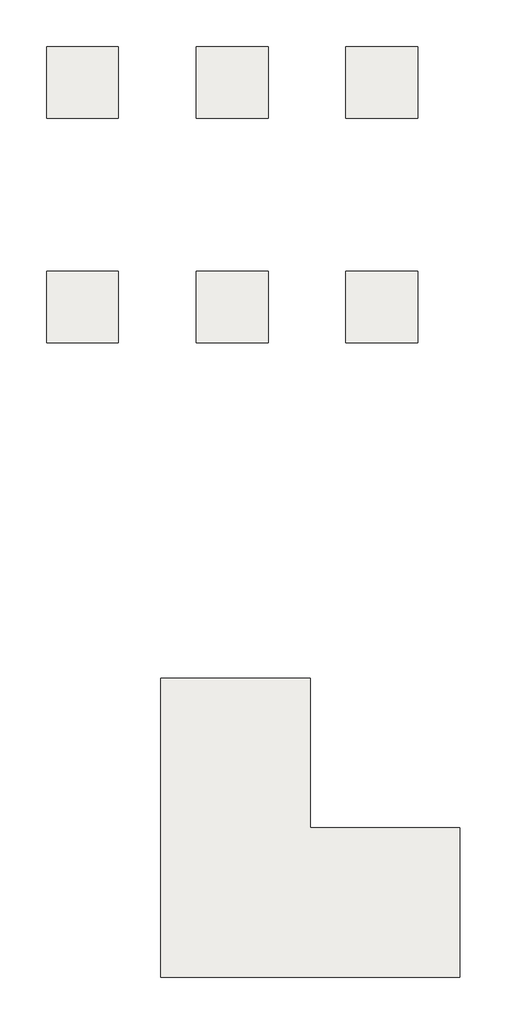
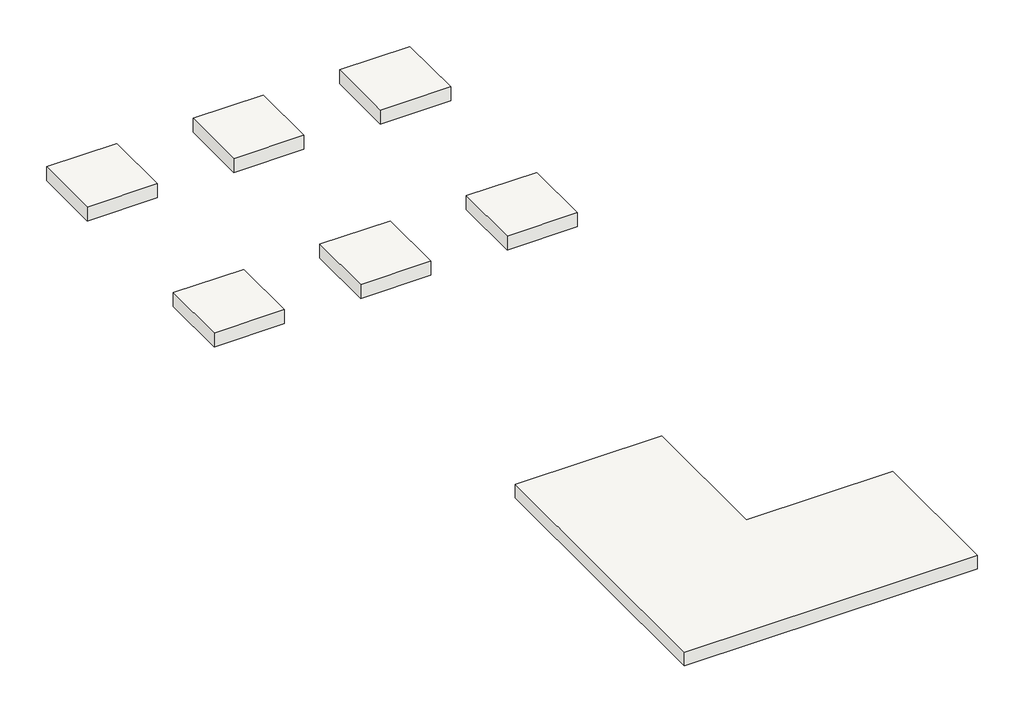
# Not in any storey: 7 slabs.
"""IFC4 building model written with IfcOpenShell, lengths in millimetres."""

import ifcopenshell
import ifcopenshell.guid

model = None  # the IFC model being written
_history = None  # IfcOwnerHistory: only IFC2X3 demands one
_inside = {}  # id of a spatial element -> (the spatial element, [elements in it])
_under = {}  # id of a project, library or spatial element -> (it, [spatial elements below it])
_declared = {}  # id of a project -> (the project, [libraries it declares])
_typed = {}  # id of a type object -> (the type object, [elements of that type])
_made_of = {}  # id of a material, layer set ... -> (it, [elements and type objects made of it])


def new_model(schema):
    """Start an empty IFC model of exactly this schema.

    Asked for "IFC4X3", IfcOpenShell would pick the latest addendum, in which some entities
    have other attributes; the version numbers below select the first issue.
    IFC2X3 requires an IfcOwnerHistory on every rooted entity: one is made here for all.
    """
    global model, _history
    if schema == "IFC4X3":
        model = ifcopenshell.file(schema_version=(4, 3, 0, 0))
    else:
        model = ifcopenshell.file(schema=schema)
    _inside.clear()
    _under.clear()
    _declared.clear()
    _typed.clear()
    _made_of.clear()
    _history = None
    if model.schema == "IFC2X3":
        org = make("IfcOrganization", Name="unknown")
        user = make(
            "IfcPersonAndOrganization",
            ThePerson=make("IfcPerson", FamilyName="unknown"),
            TheOrganization=org,
        )
        app = make(
            "IfcApplication",
            ApplicationDeveloper=org,
            Version="unknown",
            ApplicationFullName="unknown",
            ApplicationIdentifier="unknown",
        )
        _history = make(
            "IfcOwnerHistory",
            OwningUser=user,
            OwningApplication=app,
            ChangeAction="ADDED",
            CreationDate=0,
        )
    return model


def make(cls, **values):
    """One entity of the class cls with the attributes given. An attribute that is None is left unset."""
    return model.create_entity(
        cls, **{name: value for name, value in values.items() if value is not None}
    )


def rooted(cls, **values):
    """An entity with a GlobalId (a new one), such as an element, a storey or a relation."""
    return make(cls, GlobalId=ifcopenshell.guid.new(), OwnerHistory=_history, **values)


def si_unit(unit_type, name, prefix=None):
    """IfcSIUnit, for example si_unit("LENGTHUNIT", "METRE", prefix="MILLI")."""
    return make("IfcSIUnit", UnitType=unit_type, Prefix=prefix, Name=name)


def assignment(units):
    """IfcUnitAssignment: the units of a project."""
    return None if units is None else make("IfcUnitAssignment", Units=units)


def point(xyz):
    """IfcCartesianPoint."""
    return None if xyz is None else make("IfcCartesianPoint", Coordinates=xyz)


def direction(xyz):
    """IfcDirection."""
    return None if xyz is None else make("IfcDirection", DirectionRatios=xyz)


def frame(location, z_axis=None, x_axis=None):
    """IfcAxis2Placement3D, a coordinate frame: its origin and axes. An axis left out is left unset."""
    return make(
        "IfcAxis2Placement3D",
        Location=point(location),
        Axis=direction(z_axis),
        RefDirection=direction(x_axis),
    )


def origin():
    """The frame at (0, 0, 0) with its axes left unset."""
    return frame((0.0, 0.0, 0.0))


def place(relative_to, where):
    """IfcLocalPlacement: puts the frame where relative to a parent placement (None: the world)."""
    return make(
        "IfcLocalPlacement", PlacementRelTo=relative_to, RelativePlacement=where
    )


def context(
    kind, dimensions, precision=None, world=None, true_north=None, identifier=None
):
    """IfcGeometricRepresentationContext, for example the 3D "Model" context."""
    return make(
        "IfcGeometricRepresentationContext",
        ContextIdentifier=identifier,
        ContextType=kind,
        CoordinateSpaceDimension=dimensions,
        Precision=precision,
        WorldCoordinateSystem=world,
        TrueNorth=true_north,
    )


def project(units=None, contexts=None):
    """IfcProject with its units and contexts."""
    return rooted(
        "IfcProject",
        Name="project",
        RepresentationContexts=contexts,
        UnitsInContext=assignment(units),
    )


def spatial(cls, under=None, at=None, **own):
    """A site, building, storey or space (cls), placed at a placement, below another one or the project."""
    s = rooted(cls, ObjectPlacement=at, **own)
    if under is not None:
        _under.setdefault(under.id(), (under, []))[1].append(s)
    return s


def polyline(points):
    """IfcPolyline through the points."""
    return make("IfcPolyline", Points=[point(p) for p in points])


def outline(outer, holes=None, kind="AREA"):
    """IfcArbitraryClosedProfileDef: a profile drawn as a closed curve; with holes, ...WithVoids."""
    if holes is None:
        return make("IfcArbitraryClosedProfileDef", ProfileType=kind, OuterCurve=outer)
    return make(
        "IfcArbitraryProfileDefWithVoids",
        ProfileType=kind,
        OuterCurve=outer,
        InnerCurves=holes,
    )


def extrude(swept, where, along, depth):
    """IfcExtrudedAreaSolid: the profile swept, set in the frame where, extruded along a direction by depth."""
    return make(
        "IfcExtrudedAreaSolid",
        SweptArea=swept,
        Position=where,
        ExtrudedDirection=direction(along),
        Depth=depth,
    )


def shape(context_of_items, identifier, shape_type, items):
    """IfcShapeRepresentation: the items that make up one representation, for example the "Body"."""
    return make(
        "IfcShapeRepresentation",
        ContextOfItems=context_of_items,
        RepresentationIdentifier=identifier,
        RepresentationType=shape_type,
        Items=items,
    )


def source(mapping_origin, context_of_items, identifier, shape_type, items):
    """IfcRepresentationMap: a shape defined once, which mapped items show again and again."""
    return make(
        "IfcRepresentationMap",
        MappingOrigin=mapping_origin,
        MappedRepresentation=shape(context_of_items, identifier, shape_type, items),
    )


def transform(
    local_origin,
    x_axis=None,
    y_axis=None,
    z_axis=None,
    scale=None,
    scale2=None,
    scale3=None,
    uniform=True,
):
    """IfcCartesianTransformationOperator3D, or its non-uniform kind. x_axis, y_axis, z_axis: its Axis1, 2, 3."""
    if uniform:
        return make(
            "IfcCartesianTransformationOperator3D",
            Axis1=direction(x_axis),
            Axis2=direction(y_axis),
            LocalOrigin=point(local_origin),
            Scale=scale,
            Axis3=direction(z_axis),
        )
    return make(
        "IfcCartesianTransformationOperator3DnonUniform",
        Axis1=direction(x_axis),
        Axis2=direction(y_axis),
        LocalOrigin=point(local_origin),
        Scale=scale,
        Axis3=direction(z_axis),
        Scale2=scale2,
        Scale3=scale3,
    )


def mapped(mapping_source, mapping_target):
    """IfcMappedItem: shows the shape of a source again, moved by a transform."""
    return make(
        "IfcMappedItem", MappingSource=mapping_source, MappingTarget=mapping_target
    )


def made_of(thing, what):
    """Note that an element or type object is made of a material, layer set ...; save() writes the relation."""
    if what is not None:
        _made_of.setdefault(what.id(), (what, []))[1].append(thing)
    return thing


def element(
    cls,
    number,
    at=None,
    inside=None,
    cuts=None,
    type_object=None,
    material=None,
    context=None,
    identifier="Body",
    shape_type=None,
    held_by="IfcProductDefinitionShape",
    body=None,
    shapes=None,
    **own,
):
    """One element of the class cls, such as IfcWall. Its Tag is "e" and its number.

    at: its placement. inside: the storey or other place that contains it. cuts: it is an
    opening in that element (IfcRelVoidsElement). A single representation is given by context,
    identifier, shape_type and body (its items); several are given by shapes. held_by: the class
    of the entity that holds the representations. save() writes the other relations.
    """
    e = rooted(cls, Tag="e%d" % number, ObjectPlacement=at, **own)
    if body is not None:
        shapes = [shape(context, identifier, shape_type, body)]
    if shapes is not None:
        e.Representation = make(held_by, Representations=shapes)
    if inside is not None:
        _inside.setdefault(inside.id(), (inside, []))[1].append(e)
    if cuts is not None:
        rooted(
            "IfcRelVoidsElement", RelatingBuildingElement=cuts, RelatedOpeningElement=e
        )
    if type_object is not None:
        _typed.setdefault(type_object.id(), (type_object, []))[1].append(e)
    return made_of(e, material)


def aggregate(whole, parts):
    """IfcRelAggregates: a whole, such as a stair, and the parts it consists of."""
    return rooted("IfcRelAggregates", RelatingObject=whole, RelatedObjects=parts)


def save(model, path):
    """Write the relations noted so far, then the file.

    IfcRelAggregates (storeys below a building ...), IfcRelContainedInSpatialStructure (elements
    in a storey), IfcRelDefinesByType, IfcRelAssociatesMaterial and IfcRelDeclares: one each for
    every whole, place, type object, material and project.
    """
    for whole, parts in _under.values():
        aggregate(whole, parts)
    for where, things in _inside.values():
        rooted(
            "IfcRelContainedInSpatialStructure",
            RelatedElements=things,
            RelatingStructure=where,
        )
    for kind, things in _typed.values():
        rooted("IfcRelDefinesByType", RelatedObjects=things, RelatingType=kind)
    for what, things in _made_of.values():
        rooted("IfcRelAssociatesMaterial", RelatedObjects=things, RelatingMaterial=what)
    for by, libraries in _declared.values():
        rooted("IfcRelDeclares", RelatingContext=by, RelatedDefinitions=libraries)
    model.write(path)


def ft211_footing_rectangular_void_test_ft211_10000x10000x500_68336e3b(model_context):
    return source(origin(), model_context, "Body", "SweptSolid", [
        extrude(outline(polyline([(5000.0, -5000.0), (-5000.0, -5000.0), (-5000.0, 5000.0), (0.0, 5000.0), (0.0, 0.0), (5000.0, 0.0), (5000.0, -5000.0)])), frame((0.0, 0.0, -500.0), z_axis=(0.0, 0.0, 1.0), x_axis=(1.0, 0.0, 0.0)), (0.0, 0.0, 1.0), 500.0),
    ])


def ft211_2400x2400x500_5fe39465(model_context):
    return source(origin(), model_context, "Body", "SweptSolid", [
        extrude(outline(polyline([(1200.0, 1200.0), (1200.0, -1200.0), (-1200.0, -1200.0), (-1200.0, 1200.0), (1200.0, 1200.0)])), frame((0.0, 0.0, -500.0), z_axis=(0.0, 0.0, 1.0), x_axis=(1.0, 0.0, 0.0)), (0.0, 0.0, 1.0), 500.0),
    ])


model = new_model("IFC4")

# Units and contexts
model_context = context("Model", 3, world=origin())
ifc_project = project(units=[si_unit("LENGTHUNIT", "METRE", prefix="MILLI")], contexts=[model_context])

# Site, building
site = spatial("IfcSite", under=ifc_project)
building = spatial("IfcBuilding", under=site)

# Slabs
placement = place(None, origin())
ft211_footing_rectangular_void_test_ft211_10000x10000x500_shape = ft211_footing_rectangular_void_test_ft211_10000x10000x500_68336e3b(model_context)
element("IfcSlab", 1, ObjectType="FT211-Footing-Rectangular_void test : FT211_10000x10000x500_test", at=placement, inside=building, context=model_context, shape_type="MappedRepresentation", body=[
    mapped(ft211_footing_rectangular_void_test_ft211_10000x10000x500_shape, transform((7612.0, -3900.4608631, -1300.0), x_axis=(1.0, 0.0, 0.0), y_axis=(0.0, 1.0, 0.0), z_axis=(0.0, 0.0, 1.0))),
])
element("IfcSlab", 2, ObjectType="FT211-Footing-Rectangular_더미삭제 : FT211_2400x2400x500", at=placement, inside=building, context=model_context, shape_type="SweptSolid", body=[
    extrude(outline(polyline([(11200.0, 22199.5208589), (11200.0, 19799.5208589), (8800.0, 19799.5208589), (8800.0, 22199.5208589), (11200.0, 22199.5208589)])), frame((0.0, 0.0, -1800.0), z_axis=(0.0, 0.0, 1.0), x_axis=(1.0, 0.0, 0.0)), (0.0, 0.0, 1.0), 500.0),
])
element("IfcSlab", 3, ObjectType="FT211-Footing-Rectangular_더미삭제 : FT211_2400x2400x500", at=placement, inside=building, context=model_context, shape_type="SweptSolid", body=[
    extrude(outline(polyline([(6200.0, 22199.5208589), (6200.0, 19799.5208589), (3800.0, 19799.5208589), (3800.0, 22199.5208589), (6200.0, 22199.5208589)])), frame((0.0, 0.0, -1800.0), z_axis=(0.0, 0.0, 1.0), x_axis=(1.0, 0.0, 0.0)), (0.0, 0.0, 1.0), 500.0),
])
element("IfcSlab", 4, ObjectType="FT211-Footing-Rectangular_더미삭제 : FT211_2400x2400x500", at=placement, inside=building, context=model_context, shape_type="SweptSolid", body=[
    extrude(outline(polyline([(1200.0, 22199.5208589), (1200.0, 19799.5208589), (-1200.0, 19799.5208589), (-1200.0, 22199.5208589), (1200.0, 22199.5208589)])), frame((0.0, 0.0, -1800.0), z_axis=(0.0, 0.0, 1.0), x_axis=(1.0, 0.0, 0.0)), (0.0, 0.0, 1.0), 500.0),
])
element("IfcSlab", 5, ObjectType="FT211-Footing-Rectangular_더미삭제 : FT211_2400x2400x500", at=placement, inside=building, context=model_context, shape_type="SweptSolid", body=[
    extrude(outline(polyline([(1200.0, 14699.5208589), (1200.0, 12299.5208589), (-1200.0, 12299.5208589), (-1200.0, 14699.5208589), (1200.0, 14699.5208589)])), frame((0.0, 0.0, -1800.0), z_axis=(0.0, 0.0, 1.0), x_axis=(1.0, 0.0, 0.0)), (0.0, 0.0, 1.0), 500.0),
])
ft211_2400x2400x500_shape = ft211_2400x2400x500_5fe39465(model_context)
element("IfcSlab", 6, ObjectType="FT211-Footing-Rectangular_더미삭제 : FT211_2400x2400x500", at=placement, inside=building, context=model_context, shape_type="MappedRepresentation", body=[
    mapped(ft211_2400x2400x500_shape, transform((5000.0, 13499.5208589, -1300.0), x_axis=(1.0, 0.0, 0.0), y_axis=(0.0, 1.0, 0.0), z_axis=(0.0, 0.0, 1.0))),
])
element("IfcSlab", 7, ObjectType="FT211-Footing-Rectangular_더미삭제 : FT211_2400x2400x500", at=placement, inside=building, context=model_context, shape_type="MappedRepresentation", body=[
    mapped(ft211_2400x2400x500_shape, transform((10000.0, 13499.5208589, -1300.0), x_axis=(1.0, 0.0, 0.0), y_axis=(0.0, 1.0, 0.0), z_axis=(0.0, 0.0, 1.0))),
])

save(model, "model.ifc")

# Revit data of these elements
# Project information
#   Building Name = "MAIN GATE SECURITY BUILDING"
#   Project Status = "Project Status"
#   Client Name = "현대엔지니어링"
#   Project Address = "서울시 종로구 율곡로 75(계동)"
#   Project Name = "Therma Visayas Energy Project"
#   Project Number = "-"
# Grids (mm)
#   "A": line (0, 24502.793) -> (0, 11308.625)
#   "B": line (5000, 24502.793) -> (5000, 11308.625)
#   "C": line (10000, 24502.793) -> (10000, 11308.625)
#   "1": line (-3860.098, 13499.521) -> (12441.468, 13499.521)
#   "2": line (-3860.098, 20999.521) -> (12441.468, 20999.521)
# Type "FT211-Footing-Rectangular_void test : FT211_10000x10000x500_test"
#   Top bar = "D25@300"
#   Description = "UG Shallow Foundation"
#   Bottom bar = "D20@300"
#   Width = 10000 mm
#   Length = 10000 mm
#   Foundation Thickness = 500 mm
#   Structural Material [instance default] = A03AC032-00007_Structural Concrete_Type1_25MPa-30Mpa
#   Assembly Code = ""
# Type "FT211-Footing-Rectangular_더미삭제 : FT211_2400x2400x500"
#   Top bar = "D25@300"
#   Description = "UG Shallow Foundation"
#   Bottom bar = "D20@300"
#   Width = 2400 mm
#   Length = 2400 mm
#   Foundation Thickness = 500 mm
#   Structural Material [instance default] = A03AC032-00007_Structural Concrete_Type1_25MPa-30Mpa
#   Assembly Code = ""
# Element 1 (IfcSlab, "FT211-Footing-Rectangular_void test : FT211_10000x10000x500_test")
#   Comments = ""
#   Structural Material = A03AC032-00007_Structural Concrete_Type1_25MPa-30Mpa
#   Phase Created = New Construction
#   Materials on its faces: "A03AC032-00007_Structural Concrete_Type1_25MPa-30Mpa"
# Elements 2, 3, 4, 5, 6, 7 (IfcSlab, "FT211-Footing-Rectangular_더미삭제 : FT211_2400x2400x500")
#   Comments = ""
#   Mark = "F1"
#   F01) Building Name = "Main Gate House"
#   F11) Project Building Tag_Type-1 = "Common"
#   F12) Project Building Tag_Type-2 = "Common"
#   F13) Project Facility Code = "Facility Code"
#   F21) Structural Type = "Concrete"
#   F31) Standard Building Code = "IBC"
#   F41) Discipline = "AR"
#   F51) Plan Start Date-Engineering = "2015-01-01"
#   F52) Plan Finish Date-Engineering = "2015-12-31"
#   F53) Duration = "365"
#   F54) Actual Start Date-Engineering = "2015-01-01"
#   F55) Actual Finish Date-Engineering = "2015-12-31"
#   F61) Plan Start Date-Construction = "2016-08-19"
#   F62) Plan Finish Date-Construction = "2017-01-31"
#   F64) Actual Start Date-Construction = "2016-08-19"
#   F63) Duration = "202"
#   F65) Actual Finish Date-Construction = "2017-01-31"
#   F91) Plant Type = "CFPP"
#   F92) KKS Structures, Building = "UYF"
#   P01) Project Name = "TVEP"
#   P02) Project Configuration = "CFB Boiler x 2(Foster Wheeler) + STG x 2(Alstom, 150MW)"
#   P03) Project Abbreviation = "TVEP"
#   P04) Project Code = "BEPH1402"
#   P05) Project Stage = "In operation"
#   P06) Project Location = "Sito Looc, Barangay Bato, Toledo City in Philippines"
#   P07) Project Owner = "Therma Visayas, Inc."
#   P08) Project O.E = "Flour"
#   P09) Project Schedule = "ITB Issueing Date : 2013.07.30\r\nSite Survey : 2013.08.19-20\r\nBid Closing Date : 2013.11.29\r\nPreferred Bidder Notice 접수 : 2014.04.27\r\nTarget award date : 2014 05\r\nLOA 접수 : 2014.05.21\r\nSigning Ceremony : 2014.05.30"
#   P10) Basic Wind Speed = "55.6 m/s"
#   P11) Seismic = "NSCP 2010, Zone 4 (PGA : 0.4g)"
#   P12) Soil = "Sc"
#   P13) Soil Capacity = "100kN/m2"
#   P14) Pile Capacity = "PHC(D400) : 1200kN"
#   W00) Work Master Code = "A03AC032-00007"
#   W01) Work Master_Lv1 = "Concrete Work"
#   W02) Work Master_Lv2 = "Substructure Work"
#   W03) Work Master_Spec.1 = "Cement Type-1"
#   W04) Work Master_Spec.2 = "25MPa < F'c (Cylinder Strength) ≤ 30MPa"
#   W11) Activity ID = "C02AGB010"
#   W12) Activity Name = "Main Gate Security Building - Building Foundation"
#   W13) Plan Start Date = "2016-08-19"
#   W14) Plan Finish Date = "2016-09-22"
#   W15) Duration = "26"
#   W16) Actual Start Date = "2016-08-19"
#   W17) Actual Finish Date = "2016-09-22"
#   R02) Unit Price = 0
#   Structural Material = A03AC032-00007_Structural Concrete_Type1_25MPa-30Mpa
#   Phase Created = New Construction
#   Materials on its faces: "A03AC032-00007_Structural Concrete_Type1_25MPa-30Mpa"
# Materials
#   "A03AC032-00007_Structural Concrete_Type1_25MPa-30Mpa": class "Concrete", colour RGB 176 176 176, transparency 0, Keynote = "09910.A1", Description = "Reinf. Conc.", W00) Work Master Code = "A03AC032-00007", W01) Work Master_Lv1 = "Concrete Work", W02) Work Master_Lv2 = "Substructure Work", W03) Work Master_Spec.1 = "Structural Concrete", W04) Work Master_Spec.2 = "Cement Type-1", W05) Work Master_Spec.3 = "25MPa < F'c (Cylinder Strength) ≤ 30MPa", Cost = 0
